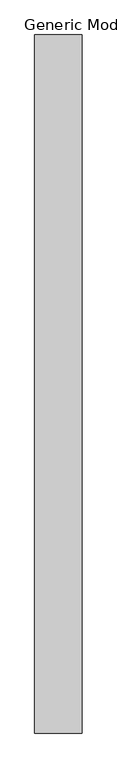
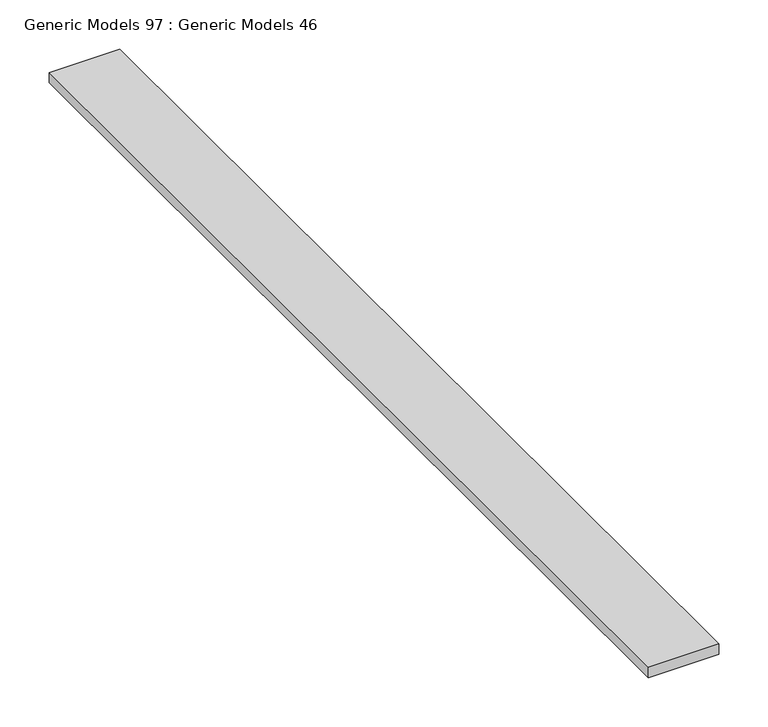
"""IFC4 building model written with IfcOpenShell, lengths in millimetres: proxy geometry, Generic Models 97 : Generic Models 46."""

from ifc_helpers import new_model, si_unit, frame, origin, place, context, project, spatial, polyline, outline, extrude, source, transform, mapped, element, save


def generic_models_97_generic_models_46_9b58c67a(model_context):
    return source(origin(), model_context, "Body", "SweptSolid", [
        extrude(outline(polyline([(48150.8590144, 0.0), (48067.9695022, 0.0), (48067.9695022, 1219.2), (48150.8590144, 1219.2), (48150.8590144, 0.0)])), frame((0.0, 0.0, 999.573933), z_axis=(0.0, 0.0, 1.0), x_axis=(1.0, 0.0, 0.0)), (0.0, 0.0, 1.0), 12.8984375),
    ])


if __name__ == "__main__":
    model = new_model("IFC4")
    model_context = context("Model", 3, world=origin())
    ifc_project = project(units=[si_unit("LENGTHUNIT", "METRE", prefix="MILLI")], contexts=[model_context])
    site = spatial("IfcSite", under=ifc_project)
    building = spatial("IfcBuilding", under=site)
    placement = place(None, origin())
    generic_models_97_generic_models_46_shape = generic_models_97_generic_models_46_9b58c67a(model_context)
    element("IfcBuildingElementProxy", 1, Name="Generic Models 97 : Generic Models 46", ObjectType="Generic Models 97 : Generic Models 46", at=placement, inside=building, context=model_context, shape_type="MappedRepresentation", body=[
        mapped(generic_models_97_generic_models_46_shape, transform((0.0, 0.0, 0.0), x_axis=(1.0, 0.0, 0.0), y_axis=(0.0, 1.0, 0.0), z_axis=(0.0, 0.0, 1.0))),
    ])
    save(model, "model.ifc")

# Revit data of these elements
# Element 1 (IfcBuildingElementProxy, "Generic Models 97 : Generic Models 46")
#   Materials on its faces: "BLOCKING - SIZE AS NEC."
# Materials
#   "BLOCKING - SIZE AS NEC.": class "Wood", colour RGB 234 198 147, transparency 0, Description = "Pinus Echinata", Cost = 0
